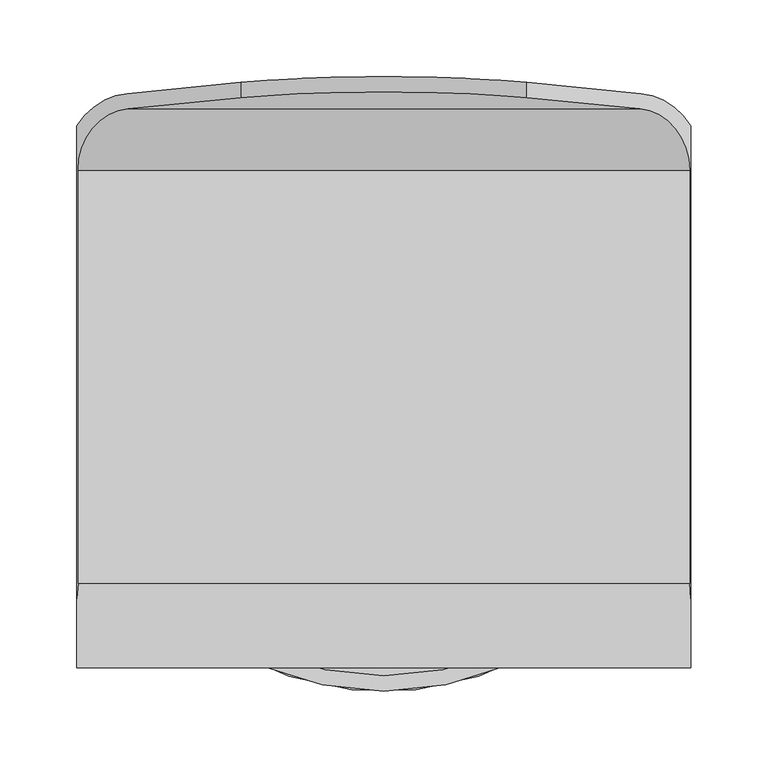
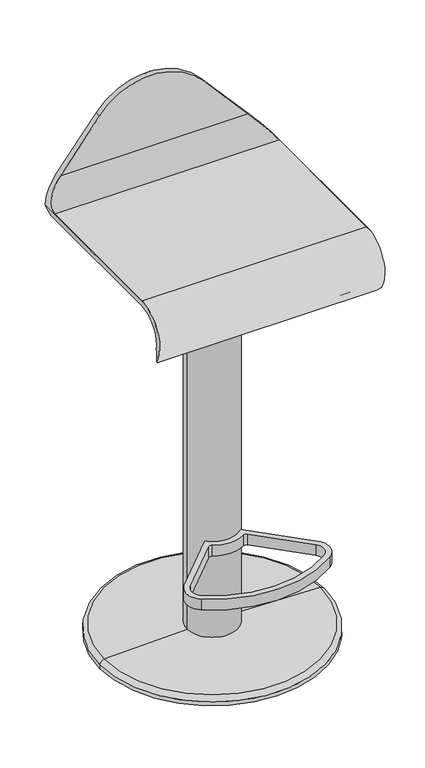
"""IFC4 building model written with IfcOpenShell, lengths in millimetres: furniture geometry, Allermuir_Surf_Stool_9179 : Allermuir_Surf_Stool_9179."""

import ifcopenshell
import ifcopenshell.guid

model = None  # the IFC model being written
_history = None  # IfcOwnerHistory: only IFC2X3 demands one
_inside = {}  # id of a spatial element -> (the spatial element, [elements in it])
_under = {}  # id of a project, library or spatial element -> (it, [spatial elements below it])
_declared = {}  # id of a project -> (the project, [libraries it declares])
_typed = {}  # id of a type object -> (the type object, [elements of that type])
_made_of = {}  # id of a material, layer set ... -> (it, [elements and type objects made of it])


def new_model(schema):
    """Start an empty IFC model of exactly this schema.

    Asked for "IFC4X3", IfcOpenShell would pick the latest addendum, in which some entities
    have other attributes; the version numbers below select the first issue.
    IFC2X3 requires an IfcOwnerHistory on every rooted entity: one is made here for all.
    """
    global model, _history
    if schema == "IFC4X3":
        model = ifcopenshell.file(schema_version=(4, 3, 0, 0))
    else:
        model = ifcopenshell.file(schema=schema)
    _inside.clear()
    _under.clear()
    _declared.clear()
    _typed.clear()
    _made_of.clear()
    _history = None
    if model.schema == "IFC2X3":
        org = make("IfcOrganization", Name="unknown")
        user = make(
            "IfcPersonAndOrganization",
            ThePerson=make("IfcPerson", FamilyName="unknown"),
            TheOrganization=org,
        )
        app = make(
            "IfcApplication",
            ApplicationDeveloper=org,
            Version="unknown",
            ApplicationFullName="unknown",
            ApplicationIdentifier="unknown",
        )
        _history = make(
            "IfcOwnerHistory",
            OwningUser=user,
            OwningApplication=app,
            ChangeAction="ADDED",
            CreationDate=0,
        )
    return model


def make(cls, **values):
    """One entity of the class cls with the attributes given. An attribute that is None is left unset."""
    return model.create_entity(
        cls, **{name: value for name, value in values.items() if value is not None}
    )


def rooted(cls, **values):
    """An entity with a GlobalId (a new one), such as an element, a storey or a relation."""
    return make(cls, GlobalId=ifcopenshell.guid.new(), OwnerHistory=_history, **values)


def si_unit(unit_type, name, prefix=None):
    """IfcSIUnit, for example si_unit("LENGTHUNIT", "METRE", prefix="MILLI")."""
    return make("IfcSIUnit", UnitType=unit_type, Prefix=prefix, Name=name)


def assignment(units):
    """IfcUnitAssignment: the units of a project."""
    return None if units is None else make("IfcUnitAssignment", Units=units)


def point(xyz):
    """IfcCartesianPoint."""
    return None if xyz is None else make("IfcCartesianPoint", Coordinates=xyz)


def direction(xyz):
    """IfcDirection."""
    return None if xyz is None else make("IfcDirection", DirectionRatios=xyz)


def frame(location, z_axis=None, x_axis=None):
    """IfcAxis2Placement3D, a coordinate frame: its origin and axes. An axis left out is left unset."""
    return make(
        "IfcAxis2Placement3D",
        Location=point(location),
        Axis=direction(z_axis),
        RefDirection=direction(x_axis),
    )


def frame_2d(location, x_axis=None):
    """IfcAxis2Placement2D, a coordinate frame in the plane: its origin and x axis."""
    return make(
        "IfcAxis2Placement2D", Location=point(location), RefDirection=direction(x_axis)
    )


def origin():
    """The frame at (0, 0, 0) with its axes left unset."""
    return frame((0.0, 0.0, 0.0))


def place(relative_to, where):
    """IfcLocalPlacement: puts the frame where relative to a parent placement (None: the world)."""
    return make(
        "IfcLocalPlacement", PlacementRelTo=relative_to, RelativePlacement=where
    )


def context(
    kind, dimensions, precision=None, world=None, true_north=None, identifier=None
):
    """IfcGeometricRepresentationContext, for example the 3D "Model" context."""
    return make(
        "IfcGeometricRepresentationContext",
        ContextIdentifier=identifier,
        ContextType=kind,
        CoordinateSpaceDimension=dimensions,
        Precision=precision,
        WorldCoordinateSystem=world,
        TrueNorth=true_north,
    )


def project(units=None, contexts=None):
    """IfcProject with its units and contexts."""
    return rooted(
        "IfcProject",
        Name="project",
        RepresentationContexts=contexts,
        UnitsInContext=assignment(units),
    )


def spatial(cls, under=None, at=None, **own):
    """A site, building, storey or space (cls), placed at a placement, below another one or the project."""
    s = rooted(cls, ObjectPlacement=at, **own)
    if under is not None:
        _under.setdefault(under.id(), (under, []))[1].append(s)
    return s


def polyline(points):
    """IfcPolyline through the points."""
    return make("IfcPolyline", Points=[point(p) for p in points])


def circle_curve(where, radius):
    """IfcCircle in the frame where."""
    return make("IfcCircle", Position=where, Radius=radius)


def ellipse_curve(where, semi_axis1, semi_axis2):
    """IfcEllipse in the frame where."""
    return make(
        "IfcEllipse", Position=where, SemiAxis1=semi_axis1, SemiAxis2=semi_axis2
    )


def trimmed(basis, trim1, trim2, sense, master):
    """IfcTrimmedCurve: the piece of a basis curve between two trims."""
    return make(
        "IfcTrimmedCurve",
        BasisCurve=basis,
        Trim1=trim1,
        Trim2=trim2,
        SenseAgreement=sense,
        MasterRepresentation=master,
    )


def segment(curve, same_sense, transition):
    """IfcCompositeCurveSegment."""
    return make(
        "IfcCompositeCurveSegment",
        Transition=transition,
        SameSense=same_sense,
        ParentCurve=curve,
    )


def composite_curve(segments, self_intersect=None):
    """IfcCompositeCurve: segments joined end to end."""
    return make("IfcCompositeCurve", Segments=segments, SelfIntersect=self_intersect)


def outline(outer, holes=None, kind="AREA"):
    """IfcArbitraryClosedProfileDef: a profile drawn as a closed curve; with holes, ...WithVoids."""
    if holes is None:
        return make("IfcArbitraryClosedProfileDef", ProfileType=kind, OuterCurve=outer)
    return make(
        "IfcArbitraryProfileDefWithVoids",
        ProfileType=kind,
        OuterCurve=outer,
        InnerCurves=holes,
    )


def extrude(swept, where, along, depth):
    """IfcExtrudedAreaSolid: the profile swept, set in the frame where, extruded along a direction by depth."""
    return make(
        "IfcExtrudedAreaSolid",
        SweptArea=swept,
        Position=where,
        ExtrudedDirection=direction(along),
        Depth=depth,
    )


def shape(context_of_items, identifier, shape_type, items):
    """IfcShapeRepresentation: the items that make up one representation, for example the "Body"."""
    return make(
        "IfcShapeRepresentation",
        ContextOfItems=context_of_items,
        RepresentationIdentifier=identifier,
        RepresentationType=shape_type,
        Items=items,
    )


def source(mapping_origin, context_of_items, identifier, shape_type, items):
    """IfcRepresentationMap: a shape defined once, which mapped items show again and again."""
    return make(
        "IfcRepresentationMap",
        MappingOrigin=mapping_origin,
        MappedRepresentation=shape(context_of_items, identifier, shape_type, items),
    )


def transform(
    local_origin,
    x_axis=None,
    y_axis=None,
    z_axis=None,
    scale=None,
    scale2=None,
    scale3=None,
    uniform=True,
):
    """IfcCartesianTransformationOperator3D, or its non-uniform kind. x_axis, y_axis, z_axis: its Axis1, 2, 3."""
    if uniform:
        return make(
            "IfcCartesianTransformationOperator3D",
            Axis1=direction(x_axis),
            Axis2=direction(y_axis),
            LocalOrigin=point(local_origin),
            Scale=scale,
            Axis3=direction(z_axis),
        )
    return make(
        "IfcCartesianTransformationOperator3DnonUniform",
        Axis1=direction(x_axis),
        Axis2=direction(y_axis),
        LocalOrigin=point(local_origin),
        Scale=scale,
        Axis3=direction(z_axis),
        Scale2=scale2,
        Scale3=scale3,
    )


def mapped(mapping_source, mapping_target):
    """IfcMappedItem: shows the shape of a source again, moved by a transform."""
    return make(
        "IfcMappedItem", MappingSource=mapping_source, MappingTarget=mapping_target
    )


def made_of(thing, what):
    """Note that an element or type object is made of a material, layer set ...; save() writes the relation."""
    if what is not None:
        _made_of.setdefault(what.id(), (what, []))[1].append(thing)
    return thing


def element(
    cls,
    number,
    at=None,
    inside=None,
    cuts=None,
    type_object=None,
    material=None,
    context=None,
    identifier="Body",
    shape_type=None,
    held_by="IfcProductDefinitionShape",
    body=None,
    shapes=None,
    **own,
):
    """One element of the class cls, such as IfcWall. Its Tag is "e" and its number.

    at: its placement. inside: the storey or other place that contains it. cuts: it is an
    opening in that element (IfcRelVoidsElement). A single representation is given by context,
    identifier, shape_type and body (its items); several are given by shapes. held_by: the class
    of the entity that holds the representations. save() writes the other relations.
    """
    e = rooted(cls, Tag="e%d" % number, ObjectPlacement=at, **own)
    if body is not None:
        shapes = [shape(context, identifier, shape_type, body)]
    if shapes is not None:
        e.Representation = make(held_by, Representations=shapes)
    if inside is not None:
        _inside.setdefault(inside.id(), (inside, []))[1].append(e)
    if cuts is not None:
        rooted(
            "IfcRelVoidsElement", RelatingBuildingElement=cuts, RelatedOpeningElement=e
        )
    if type_object is not None:
        _typed.setdefault(type_object.id(), (type_object, []))[1].append(e)
    return made_of(e, material)


def aggregate(whole, parts):
    """IfcRelAggregates: a whole, such as a stair, and the parts it consists of."""
    return rooted("IfcRelAggregates", RelatingObject=whole, RelatedObjects=parts)


def save(model, path):
    """Write the relations noted so far, then the file.

    IfcRelAggregates (storeys below a building ...), IfcRelContainedInSpatialStructure (elements
    in a storey), IfcRelDefinesByType, IfcRelAssociatesMaterial and IfcRelDeclares: one each for
    every whole, place, type object, material and project.
    """
    for whole, parts in _under.values():
        aggregate(whole, parts)
    for where, things in _inside.values():
        rooted(
            "IfcRelContainedInSpatialStructure",
            RelatedElements=things,
            RelatingStructure=where,
        )
    for kind, things in _typed.values():
        rooted("IfcRelDefinesByType", RelatedObjects=things, RelatingType=kind)
    for what, things in _made_of.values():
        rooted("IfcRelAssociatesMaterial", RelatedObjects=things, RelatingMaterial=what)
    for by, libraries in _declared.values():
        rooted("IfcRelDeclares", RelatingContext=by, RelatedDefinitions=libraries)
    model.write(path)


def plane_surface(at):
    """IfcPlane: the flat surface through the origin of the frame at, square to its z axis."""
    return make("IfcPlane", Position=at)


def cylinder_surface(at, radius):
    """IfcCylindricalSurface: all points at the distance radius from the z axis of the frame at."""
    return make("IfcCylindricalSurface", Position=at, Radius=radius)


def revolved_surface(curve, axis_point, axis_direction):
    """IfcSurfaceOfRevolution: the curve turned about the line through axis_point along axis_direction."""
    return make(
        "IfcSurfaceOfRevolution",
        SweptCurve=make("IfcArbitraryOpenProfileDef", ProfileType="CURVE", Curve=curve),
        AxisPosition=make("IfcAxis1Placement", Location=point(axis_point), Axis=direction(axis_direction)),
    )


def advanced_brep(points, edges, surfaces, faces):
    """IfcAdvancedBrep: a solid bounded by faces that lie on surfaces and meet in shared edges.

    An edge is (start, end): straight between two places in points (the first is 0);
    or (start, end, curve); or (start, end, curve, False) where it runs against its curve.
    A face is (place in surfaces, loops), or (place, loops, False) where it looks against
    its surface's normal. A loop lists edges by number (the first is 1), with a minus sign
    where the edge is run from its end to its start. The first loop is the outer one.
    """
    corners = [point(p) for p in points]
    vertices = [make("IfcVertexPoint", VertexGeometry=c) for c in corners]
    made = []
    for start, end, *more in edges:
        made.append(
            make(
                "IfcEdgeCurve",
                EdgeStart=vertices[start],
                EdgeEnd=vertices[end],
                EdgeGeometry=more[0] if more else make("IfcPolyline", Points=[corners[start], corners[end]]),
                SameSense=more[1] if len(more) > 1 else True,
            )
        )
    hull = []
    for where, loops, *sense in faces:
        bounds = []
        for j, loop in enumerate(loops):
            ring = [make("IfcOrientedEdge", EdgeElement=made[abs(k) - 1], Orientation=k > 0) for k in loop]
            bounds.append(
                make(
                    "IfcFaceOuterBound" if j == 0 else "IfcFaceBound",
                    Bound=make("IfcEdgeLoop", EdgeList=ring),
                    Orientation=True,
                )
            )
        hull.append(make("IfcAdvancedFace", Bounds=bounds, FaceSurface=surfaces[where], SameSense=sense[0] if sense else True))
    return make("IfcAdvancedBrep", Outer=make("IfcClosedShell", CfsFaces=hull))


def furniture_eb32228c(model_context):
    return source(origin(), model_context, "Body", "SolidModel", [
        extrude(outline(composite_curve([segment(trimmed(circle_curve(frame_2d((231.753449, 164.0039103)), 3.0), [point((229.7688585, 166.2536659))], [point((233.8747694, 166.1252306))], False, "CARTESIAN"), True, "CONTINUOUS"), segment(polyline([(233.8747694, 166.1252306), (318.3215957, 81.6784043)]), True, "CONTINUOUS"), segment(trimmed(circle_curve(frame_2d((297.1083922, 60.4652009)), 30.0), [point((318.3215957, 81.6784043))], [point((314.2451673, 35.8414128))], False, "CARTESIAN"), True, "CONTINUOUS"), segment(trimmed(circle_curve(frame_2d((200.0, 200.0)), 200.0), [point((314.2451673, 35.8414128))], [point((85.7548327, 35.8414128))], False, "CARTESIAN"), True, "CONTINUOUS"), segment(trimmed(circle_curve(frame_2d((102.8916078, 60.4652009)), 30.0), [point((85.7548327, 35.8414128))], [point((81.6784043, 81.6784043))], False, "CARTESIAN"), True, "CONTINUOUS"), segment(polyline([(81.6784043, 81.6784043), (166.1252306, 166.1252306)]), True, "CONTINUOUS"), segment(trimmed(circle_curve(frame_2d((168.246551, 164.0039103)), 3.0), [point((166.1252306, 166.1252306))], [point((170.2311415, 166.2536659))], False, "CARTESIAN"), True, "CONTINUOUS"), segment(trimmed(circle_curve(frame_2d((200.0, 200.0)), 45.0), [point((170.2311415, 166.2536659))], [point((229.7688585, 166.2536659))], True, "CARTESIAN"), True, "CONTINUOUS")], self_intersect=False), holes=[composite_curve([segment(polyline([(165.991876, 151.8497404), (88.7494721, 74.6073365)]), True, "CONTINUOUS"), segment(trimmed(circle_curve(frame_2d((102.8916078, 60.4652009)), 20.0), [point((88.7494721, 74.6073365))], [point((91.467091, 44.0493422))], True, "CARTESIAN"), True, "CONTINUOUS"), segment(trimmed(circle_curve(frame_2d((200.0, 200.0)), 190.0), [point((91.467091, 44.0493422))], [point((308.532909, 44.0493422))], True, "CARTESIAN"), True, "CONTINUOUS"), segment(trimmed(circle_curve(frame_2d((297.1083922, 60.4652009)), 20.0), [point((308.532909, 44.0493422))], [point((311.2505279, 74.6073365))], True, "CARTESIAN"), True, "CONTINUOUS"), segment(polyline([(311.2505279, 74.6073365), (234.008124, 151.8497404)]), True, "CONTINUOUS"), segment(trimmed(circle_curve(frame_2d((230.4725901, 148.3142065)), 5.0), [point((234.008124, 151.8497404))], [point((227.9332076, 152.6213559))], True, "CARTESIAN"), True, "CONTINUOUS"), segment(trimmed(circle_curve(frame_2d((200.0, 200.0)), 55.0), [point((227.9332076, 152.6213559))], [point((172.0667924, 152.6213559))], False, "CARTESIAN"), True, "CONTINUOUS"), segment(trimmed(circle_curve(frame_2d((169.5274099, 148.3142065)), 5.0), [point((172.0667924, 152.6213559))], [point((165.991876, 151.8497404))], True, "CARTESIAN"), True, "CONTINUOUS")], self_intersect=False)]), frame((0.0, 0.0, 180.0), z_axis=(0.0, 0.0, 1.0), x_axis=(1.0, 0.0, 0.0)), (0.0, 0.0, 1.0), 20.0),
        advanced_brep(
        [(245.0, 200.0, 20.0), (155.0, 200.0, 20.0), (155.0, 200.0, 0.0), (245.0, 200.0, 0.0), (392.041203, 200.0, 15.2567354), (7.958797, 200.0, 15.2567354), (400.0, 200.0, 0.0), (0.0, 200.0, 0.0), (0.0, 200.0, 7.0370632), (400.0, 200.0, 7.0370632)],
        [
            (0, 1, circle_curve(frame((200.0, 200.0, 20.0), z_axis=(0.0, 0.0, 1.0), x_axis=(-1.0, 0.0, 0.0)), 45.0)),
            (1, 2),
            (2, 3, circle_curve(frame((200.0, 200.0, 0.0), z_axis=(0.0, 0.0, -1.0), x_axis=(-1.0, 0.0, 0.0)), 45.0)),
            (3, 0),
            (1, 0, circle_curve(frame((200.0, 200.0, 20.0), z_axis=(0.0, 0.0, 1.0), x_axis=(-1.0, 0.0, 0.0)), 45.0)),
            (3, 2, circle_curve(frame((200.0, 200.0, 0.0), z_axis=(0.0, 0.0, -1.0), x_axis=(-1.0, 0.0, 0.0)), 45.0)),
            (4, 5, circle_curve(frame((200.0, 200.0, 15.2567354), z_axis=(0.0, 0.0, 1.0), x_axis=(-1.0, 0.0, 0.0)), 192.041203)),
            (5, 1),
            (0, 4),
            (5, 4, circle_curve(frame((200.0, 200.0, 15.2567354), z_axis=(0.0, 0.0, 1.0), x_axis=(-1.0, 0.0, 0.0)), 192.041203)),
            (6, 7, circle_curve(frame((200.0, 200.0, 0.0), z_axis=(0.0, 0.0, 1.0), x_axis=(-1.0, 0.0, 0.0)), 200.0)),
            (7, 8),
            (8, 9, circle_curve(frame((200.0, 200.0, 7.0370632), z_axis=(0.0, 0.0, -1.0), x_axis=(-1.0, 0.0, 0.0)), 200.0)),
            (9, 6),
            (7, 6, circle_curve(frame((200.0, 200.0, 0.0), z_axis=(0.0, 0.0, 1.0), x_axis=(-1.0, 0.0, 0.0)), 200.0)),
            (9, 8, circle_curve(frame((200.0, 200.0, 7.0370632), z_axis=(0.0, 0.0, -1.0), x_axis=(-1.0, 0.0, 0.0)), 200.0)),
            (2, 7),
            (6, 3),
            (8, 5, circle_curve(frame((8.2239477, 200.0, 7.0370632), z_axis=(0.0, 1.0, 0.0), x_axis=(1.0, 0.0, 0.0)), 8.2239477)),
            (4, 9, circle_curve(frame((391.7760523, 200.0, 7.0370632), z_axis=(0.0, 1.0, 0.0), x_axis=(-1.0, 0.0, 0.0)), 8.2239477)),
        ],
        [
            revolved_surface(polyline([(155.0, 200.0, 0.0), (155.0, 200.0, 20.0)]), (200.0, 200.0, 2438.4), (0.0, 0.0, -1.0)),
            revolved_surface(polyline([(155.0, 200.0, 20.0), (7.958797, 200.0, 15.2567354)]), (200.0, 200.0, 2438.4), (0.0, 0.0, -1.0)),
            cylinder_surface(frame((200.0, 200.0, 2438.4), z_axis=(0.0, 0.0, -1.0), x_axis=(-1.0, 0.0, 0.0)), 200.0),
            plane_surface(frame((200.0, 200.0, 0.0), z_axis=(0.0, 0.0, -1.0), x_axis=(-1.0, 0.0, 0.0))),
            revolved_surface(trimmed(ellipse_curve(frame((8.2239477, 200.0, 7.0370632), z_axis=(0.0, -1.0, 0.0), x_axis=(1.0, 0.0, 0.0)), 8.2239477, 8.2239477), [point((7.958797, 200.0, 15.2567354))], [point((0.0, 200.0, 7.0370632))], True, "CARTESIAN"), (200.0, 200.0, 2438.4), (0.0, 0.0, -1.0)),
        ],
        [
            (0, [[1, 2, 3, 4]]),
            (0, [[5, -4, 6, -2]]),
            (1, [[7, 8, -1, 9]]),
            (1, [[10, -9, -5, -8]]),
            (2, [[11, 12, 13, 14]]),
            (2, [[15, -14, 16, -12]]),
            (3, [[-3, 17, -11, 18]]),
            (3, [[-6, -18, -15, -17]]),
            (4, [[-13, 19, -7, 20]]),
            (4, [[-16, -20, -10, -19]]),
        ],
    ),
        advanced_brep(
        [(155.0, 200.0, 0.0), (245.0, 200.0, 0.0), (245.0, 200.0, 579.3900193), (155.0, 200.0, 579.3900193)],
        [
            (0, 1, circle_curve(frame((200.0, 200.0, 0.0), z_axis=(0.0, 0.0, -1.0), x_axis=(1.0, 0.0, 0.0)), 45.0)),
            (1, 0, circle_curve(frame((200.0, 200.0, 0.0), z_axis=(0.0, 0.0, -1.0), x_axis=(1.0, 0.0, 0.0)), 45.0)),
            (1, 2),
            (2, 3, ellipse_curve(frame((200.0, 200.0, 579.3900193), z_axis=(0.0, -0.5399439781834036, -0.8417009566487852), x_axis=(0.0, -0.8417009566487852, 0.5399439781834037)), 53.4631684, 45.0)),
            (3, 0),
            (3, 2, ellipse_curve(frame((200.0, 200.0, 579.3900193), z_axis=(0.0, -0.5399439781834036, -0.8417009566487852), x_axis=(0.0, -0.8417009566487852, 0.5399439781834037)), 53.4631684, 45.0)),
        ],
        [
            plane_surface(frame((245.0, 200.0, 0.0), z_axis=(0.0, 0.0, -1.0), x_axis=(0.0, -1.0, 0.0))),
            cylinder_surface(frame((200.0, 200.0, 0.0), z_axis=(0.0, 0.0, 1.0), x_axis=(1.0, 0.0, 0.0)), 45.0),
            plane_surface(frame((319.4506408, 140.0142682, 617.8703542), z_axis=(0.0, 0.5399439781834036, 0.8417009566487852), x_axis=(-1.0, 0.0, 0.0))),
        ],
        [
            (0, [[1, 2]]),
            (1, [[-2, 3, 4, 5]]),
            (1, [[-1, -5, 6, -3]]),
            (2, [[-4, -6]]),
        ],
    ),
        advanced_brep(
        [(400.0, 70.0919848, 760.0), (400.0, 339.3103685, 760.0), (400.0, 368.030606, 769.0714286), (400.0, 60.0281579, 769.0714286), (400.0, 25.0919848, 683.3772234), (400.0, 25.0919848, 705.2464075), (400.0, 26.1617284, 705.2464075), (0.0, 339.3103685, 760.0), (0.0, 70.0919848, 760.0), (0.0, 26.1617284, 705.2464075), (0.0, 25.0919848, 705.2464075), (0.0, 25.0919848, 683.3772234), (0.0, 60.0281579, 769.0714286), (0.0, 368.030606, 769.0714286), (367.2640038, 389.1201034, 805.6422129), (32.7359962, 389.1201034, 805.6422129), (106.8635277, 396.3651308, 888.4532553), (195.445222, 400.0, 930.0), (204.554778, 400.0, 930.0), (293.1364723, 396.3651308, 888.4532553), (33.5161627, 379.1581564, 806.5137703), (366.4838373, 379.1581564, 806.5137703), (293.1364723, 386.3269325, 888.4532553), (106.8635277, 386.3269325, 888.4532553), (0.831202, 339.3103685, 770.0), (399.168798, 339.3103685, 770.0), (0.831202, 70.0919848, 770.0), (399.168798, 70.0919848, 770.0), (11.5316988, 40.395066, 668.7064474), (388.4683012, 40.395066, 668.7064474), (156.0750469, 232.2105677, 545.6584406), (243.9249531, 232.2105677, 545.6584406), (245.0, 200.0, 566.3212448), (155.0, 200.0, 566.3212448), (15.6004685, 45.7945058, 677.123457), (384.3995315, 45.7945058, 677.123457), (243.9249531, 232.2105677, 557.5391447), (156.0750469, 232.2105677, 557.5391447), (155.0, 200.0, 578.2019489), (245.0, 200.0, 578.2019489), (399.1938904, 26.1617284, 705.2464075), (0.8061096, 26.1617284, 705.2464075)],
        [
            (0, 1),
            (1, 2, circle_curve(frame((400.0, 339.3103685, 810.0), z_axis=(1.0, 0.0, 0.0), x_axis=(0.0, -1.0, 0.0)), 50.0)),
            (2, 3),
            (3, 4, circle_curve(frame((400.0, 70.0919848, 715.0), z_axis=(1.0, 0.0, 0.0), x_axis=(0.0, -1.0, 0.0)), 55.0)),
            (4, 5),
            (5, 6),
            (6, 0, circle_curve(frame((400.0, 70.0919848, 715.0), z_axis=(-1.0, 0.0, 0.0), x_axis=(0.0, -1.0, 0.0)), 45.0)),
            (7, 8),
            (8, 9, circle_curve(frame((0.0, 70.0919848, 715.0), z_axis=(1.0, 0.0, 0.0), x_axis=(0.0, -1.0, 0.0)), 45.0)),
            (9, 10),
            (10, 11),
            (11, 12, circle_curve(frame((0.0, 70.0919848, 715.0), z_axis=(-1.0, 0.0, 0.0), x_axis=(0.0, -1.0, 0.0)), 55.0)),
            (12, 13),
            (13, 7, circle_curve(frame((0.0, 339.3103685, 810.0), z_axis=(-1.0, 0.0, 0.0), x_axis=(0.0, -1.0, 0.0)), 50.0)),
            (14, 15),
            (15, 16),
            (16, 17, ellipse_curve(frame((200.0, 389.0711796, 805.0830116), z_axis=(0.0, 0.9961946980917454, -0.08715574274765918), x_axis=(0.0, 0.08715574274765936, 0.9961946980917454)), 125.4774797, 125.0)),
            (17, 18),
            (18, 19, ellipse_curve(frame((200.0, 389.0711796, 805.0830116), z_axis=(0.0, 0.9961946980917454, -0.08715574274765918), x_axis=(0.0, 0.08715574274765936, 0.9961946980917454)), 125.4774797, 125.0)),
            (19, 14),
            (17, 18, ellipse_curve(frame((200.0, 1827.8077112, 805.0830116), z_axis=(0.0, 0.0871557427476659, 0.9961946980917449), x_axis=(0.0, 0.9961946980917449, -0.0871557427476659)), 1434.2141557, 125.0)),
            (20, 21),
            (21, 22),
            (22, 23, ellipse_curve(frame((200.0, 379.0329813, 805.0830116), z_axis=(0.0, -0.9961946980917454, 0.08715574274765944), x_axis=(0.0, 0.0871557427476591, 0.9961946980917454)), 125.4774797, 125.0)),
            (23, 20),
            (20, 24, ellipse_curve(frame((36.6368286, 339.3103685, 810.0), z_axis=(-0.745091778044962, 0.0, 0.6669619496566481), x_axis=(-0.666961949656648, 0.0, -0.745091778044962)), 53.6846616, 40.0)),
            (24, 25),
            (25, 21, ellipse_curve(frame((363.3631714, 339.3103685, 810.0), z_axis=(0.7450917780449817, 0.0, 0.6669619496566261), x_axis=(-0.6669619496566259, 0.0, 0.7450917780449818)), 53.6846616, 40.0)),
            (24, 26),
            (26, 27),
            (27, 25),
            (0, 8),
            (7, 1),
            (13, 15, ellipse_curve(frame((36.6368286, 339.3103685, 810.0), z_axis=(0.745091778044962, 0.0, -0.6669619496566481), x_axis=(0.666961949656648, 0.0, 0.745091778044962)), 67.1058271, 50.0)),
            (14, 2, ellipse_curve(frame((363.3631714, 339.3103685, 810.0), z_axis=(-0.7450917780449817, 0.0, -0.6669619496566261), x_axis=(0.6669619496566259, 0.0, -0.7450917780449818)), 67.1058271, 50.0)),
            (19, 22),
            (27, 3, ellipse_curve(frame((448.4015345, 70.0919848, 715.0), z_axis=(0.7450917780449817, 0.0, 0.6669619496566261), x_axis=(0.6669619496566259, 0.0, -0.7450917780449818)), 73.8164098, 55.0)),
            (23, 16),
            (12, 26, ellipse_curve(frame((-48.4015345, 70.0919848, 715.0), z_axis=(-0.745091778044962, 0.0, 0.6669619496566481), x_axis=(0.666961949656648, 0.0, 0.745091778044962)), 73.8164098, 55.0)),
            (11, 28, ellipse_curve(frame((33.9099323, 70.0919848, 715.0), z_axis=(0.798635510047292, -0.6018150231520493, 0.0), x_axis=(0.6018150231520494, 0.7986355100472919, 0.0)), 68.8674612, 55.0)),
            (28, 29),
            (29, 4, ellipse_curve(frame((366.0900677, 70.0919848, 715.0), z_axis=(-0.798635510047292, -0.6018150231520495, 0.0), x_axis=(0.6018150231520493, -0.7986355100472922, 0.0)), 68.8674612, 55.0)),
            (28, 30),
            (30, 31, ellipse_curve(frame((200.0, 199.1107414, 566.8916966), z_axis=(0.0, -0.5399439781834032, -0.8417009566487854), x_axis=(0.0, 0.8417009566487854, -0.5399439781834033)), 65.3438725, 55.0)),
            (31, 29),
            (32, 33, ellipse_curve(frame((200.0, 200.0, 566.3212448), z_axis=(0.0, 0.5399439781834032, 0.8417009566487854), x_axis=(0.0, -0.8417009566487854, 0.5399439781834033)), 53.4631684, 45.0)),
            (33, 32, ellipse_curve(frame((200.0, 200.0, 566.3212448), z_axis=(0.0, 0.5399439781834032, 0.8417009566487854), x_axis=(0.0, -0.8417009566487854, 0.5399439781834033)), 53.4631684, 45.0)),
            (34, 35),
            (35, 36),
            (36, 37, ellipse_curve(frame((200.0, 199.1107414, 578.7724007), z_axis=(0.0, 0.5399439781834033, 0.8417009566487854), x_axis=(0.0, 0.8417009566487854, -0.5399439781834032)), 65.3438725, 55.0)),
            (37, 34),
            (38, 39, ellipse_curve(frame((200.0, 200.0, 578.2019489), z_axis=(0.0, -0.5399439781834033, -0.8417009566487854), x_axis=(0.0, -0.8417009566487854, 0.5399439781834032)), 53.4631684, 45.0)),
            (39, 38, ellipse_curve(frame((200.0, 200.0, 578.2019489), z_axis=(0.0, -0.5399439781834033, -0.8417009566487854), x_axis=(0.0, -0.8417009566487854, 0.5399439781834032)), 53.4631684, 45.0)),
            (6, 40),
            (40, 35, ellipse_curve(frame((366.0900677, 70.0919848, 715.0), z_axis=(0.798635510047292, 0.6018150231520495, 0.0), x_axis=(-0.6018150231520493, 0.7986355100472922, 0.0)), 56.3461046, 45.0)),
            (34, 41, ellipse_curve(frame((33.9099323, 70.0919848, 715.0), z_axis=(-0.798635510047292, 0.6018150231520493, 0.0), x_axis=(-0.6018150231520494, -0.7986355100472919, 0.0)), 56.3461046, 45.0)),
            (41, 9),
            (5, 40),
            (41, 10),
            (30, 37),
            (36, 31),
            (32, 39),
            (38, 33),
        ],
        [
            plane_surface(frame((400.0, 400.0, 930.0), z_axis=(1.0, 0.0, 0.0), x_axis=(0.0, 0.08715574274765918, 0.9961946980917454))),
            plane_surface(frame((0.0, 400.0, 930.0), z_axis=(-1.0, 0.0, 0.0), x_axis=(0.0, -0.08715574274765918, -0.9961946980917454))),
            plane_surface(frame((400.0, 389.1201034, 805.6422129), z_axis=(0.0, 0.9961946980917454, -0.08715574274765918), x_axis=(-1.0, 0.0, 0.0))),
            plane_surface(frame((400.0, 400.0, 930.0), z_axis=(0.0, 0.0871557427476659, 0.9961946980917449), x_axis=(-1.0, 0.0, 0.0))),
            plane_surface(frame((400.0, 390.038053, 930.8715574), z_axis=(0.0, -0.9961946980917454, 0.08715574274765944), x_axis=(-1.0, 0.0, 0.0))),
            revolved_surface(polyline([(0.831202, 299.3103685, 810.0), (399.168798, 299.3103685, 810.0)]), (0.0, 339.3103685, 810.0), (-1.0, 0.0, 0.0)),
            plane_surface(frame((400.0, 339.3103685, 770.0), z_axis=(0.0, 0.0, 1.0), x_axis=(-1.0, 0.0, 0.0))),
            plane_surface(frame((400.0, 70.0919848, 760.0), z_axis=(0.0, 0.0, -1.0), x_axis=(-1.0, 0.0, 0.0))),
            cylinder_surface(frame((0.0, 339.3103685, 810.0), z_axis=(1.0, 0.0, 0.0), x_axis=(0.0, -1.0, 0.0)), 50.0),
            plane_surface(frame((293.1364723, -206.7636844, 888.4532553), z_axis=(0.7450917780449817, 0.0, 0.6669619496566261), x_axis=(0.0, 1.0, 0.0))),
            plane_surface(frame((-8.1202046, -206.7636844, 760.0), z_axis=(-0.745091778044962, 0.0, 0.6669619496566481), x_axis=(0.0, 1.0, 0.0))),
            cylinder_surface(frame((200.0, 480.8963376, 805.0830116), z_axis=(0.0, 1.0, 0.0), x_axis=(-1.0, 0.0, 0.0)), 125.0),
            cylinder_surface(frame((0.0, 70.0919848, 715.0), z_axis=(1.0, 0.0, 0.0), x_axis=(0.0, -1.0, 0.0)), 55.0),
            plane_surface(frame((400.0, 40.395066, 668.7064474), z_axis=(0.0, -0.5399439781834032, -0.8417009566487854), x_axis=(-1.0, 0.0, 0.0))),
            plane_surface(frame((400.0, 272.006426, 532.0104413), z_axis=(0.0, 0.5399439781834033, 0.8417009566487854), x_axis=(-1.0, 0.0, 0.0))),
            revolved_surface(polyline([(0.0, 25.091984800000006, 715.0), (400.0, 25.091984800000006, 715.0)]), (0.0, 70.0919848, 715.0), (-1.0, 0.0, 0.0)),
            plane_surface(frame((255.0, 199.1107414, 705.2464075), z_axis=(0.0, 0.0, -1.0), x_axis=(0.0, -1.0, 0.0))),
            cylinder_surface(frame((200.0, 199.1107414, 482.1686256), z_axis=(0.0, 0.0, -1.0), x_axis=(1.0, 0.0, 0.0)), 55.0),
            plane_surface(frame((243.9249531, 232.2105677, 705.2464075), z_axis=(0.798635510047292, 0.6018150231520495, 0.0), x_axis=(0.0, 0.0, -1.0))),
            plane_surface(frame((0.0, 25.0919848, 705.2464075), z_axis=(-0.798635510047292, 0.6018150231520493, 0.0), x_axis=(0.0, 0.0, -1.0))),
            revolved_surface(polyline([(245.0, 200.0, 607.0690647321853), (245.0, 200.0, 537.4541289678148)]), (200.0, 200.0, 482.1686256), (0.0, 0.0, 1.0)),
        ],
        [
            (0, [[1, 2, 3, 4, 5, 6, 7]]),
            (1, [[8, 9, 10, 11, 12, 13, 14]]),
            (2, [[15, 16, 17, 18, 19, 20]]),
            (3, [[-18, 21]]),
            (4, [[22, 23, 24, 25]]),
            (5, [[-22, 26, 27, 28]]),
            (6, [[-27, 29, 30, 31]]),
            (7, [[-1, 32, -8, 33]]),
            (8, [[-33, -14, 34, -15, 35, -2]]),
            (9, [[36, -23, -28, -31, 37, -3, -35, -20]]),
            (10, [[38, -16, -34, -13, 39, -29, -26, -25]]),
            (11, [[-36, -19, -21, -17, -38, -24]]),
            (12, [[-30, -39, -12, 40, 41, 42, -4, -37]]),
            (13, [[-41, 43, 44, 45], [46, 47]]),
            (14, [[48, 49, 50, 51], [52, 53]]),
            (15, [[-32, -7, 54, 55, -48, 56, 57, -9]]),
            (16, [[58, -54, -6]]),
            (16, [[59, -10, -57]]),
            (17, [[60, -50, 61, -44]]),
            (18, [[-58, -5, -42, -45, -61, -49, -55]]),
            (19, [[-59, -56, -51, -60, -43, -40, -11]]),
            (20, [[62, -52, 63, -46]]),
            (20, [[-62, -47, -63, -53]]),
        ],
    ),
    ])


if __name__ == "__main__":
    model = new_model("IFC4")
    model_context = context("Model", 3, world=origin())
    ifc_project = project(units=[si_unit("LENGTHUNIT", "METRE", prefix="MILLI")], contexts=[model_context])
    site = spatial("IfcSite", under=ifc_project)
    building = spatial("IfcBuilding", under=site)
    placement = place(None, origin())
    furniture_shape = furniture_eb32228c(model_context)
    element("IfcFurniture", 1, ObjectType="Allermuir_Surf_Stool_9179 : Allermuir_Surf_Stool_9179", at=placement, inside=building, context=model_context, shape_type="MappedRepresentation", body=[
        mapped(furniture_shape, transform((0.0, 0.0, 0.0), x_axis=(1.0, 0.0, 0.0), y_axis=(0.0, 1.0, 0.0), z_axis=(0.0, 0.0, 1.0))),
    ])
    save(model, "model.ifc")

# Revit data of these elements
# Type "Allermuir_Surf_Stool_9179 : Allermuir_Surf_Stool_9179"
#   Support = chrome
#   Seat = orange paint
#   Base = chrome
#   Default Elevation = 0
# Element 1 (IfcFurniture, "Allermuir_Surf_Stool_9179 : Allermuir_Surf_Stool_9179")
#   Materials on its faces: "chrome", "orange paint"
# Materials
#   "chrome": class "Metal", colour RGB 244 244 244, transparency 0
#   "orange paint": class "Paint", colour RGB 248 199 146, transparency 0, Cost = 0
